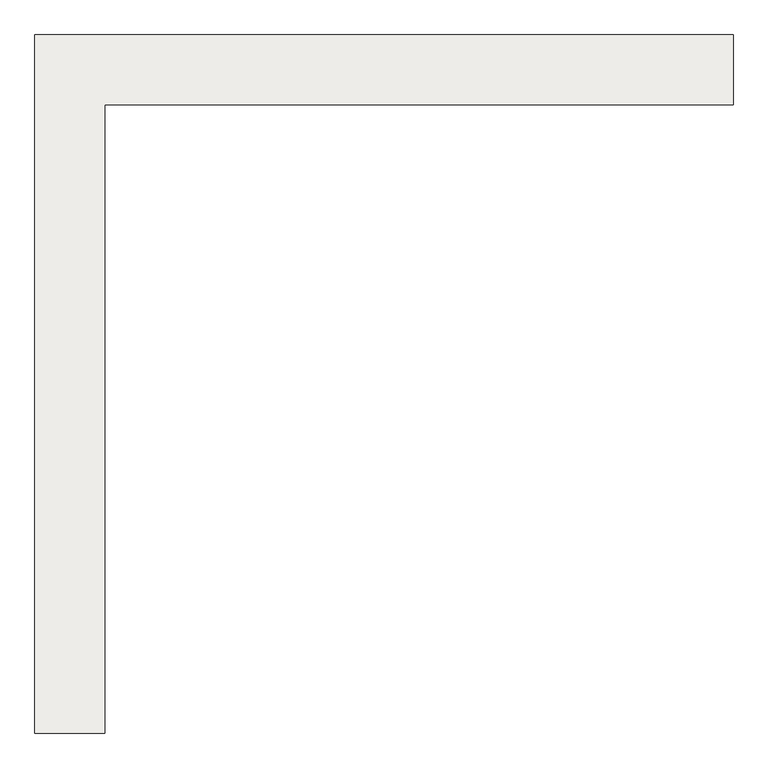
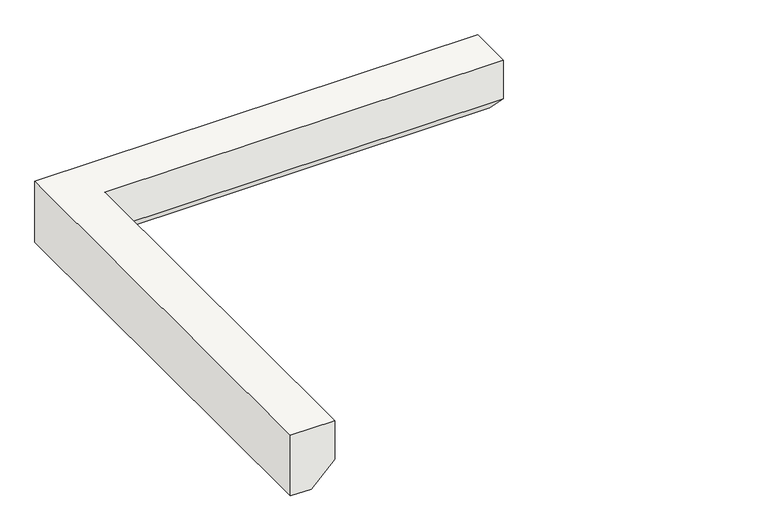
"""IFC4 building model written with IfcOpenShell, lengths in millimetres: slab geometry, hslab edge test : hslab edge test 1."""

from ifc_helpers import new_model, si_unit, origin, place, context, project, spatial, faceted_brep, source, transform, mapped, element, save


def slab_4663229b(model_context):
    return source(origin(), model_context, "Body", "Brep", [
        faceted_brep([(-959.1559606, 19799.5208589, -2020.0), (-959.1559606, 19799.5208589, -1800.0), (-1200.0, 19799.5208589, -1800.0), (-1200.0, 19799.5208589, -2147.2792206), (-1086.4351812, 19799.5208589, -2147.2792206), (-959.1559606, 21958.6768195, -2020.0), (-959.1559606, 21958.6768195, -1800.0), (1200.0, 21958.6768195, -1800.0), (1200.0, 22199.5208589, -1800.0), (-1200.0, 22199.5208589, -1800.0), (-1200.0, 22199.5208589, -2147.2792206), (1200.0, 22199.5208589, -2147.2792206), (1200.0, 22085.9560401, -2147.2792206), (-1086.4351812, 22085.9560401, -2147.2792206), (1200.0, 21958.6768195, -2020.0)], [[[0, 1, 2, 3, 4]], [[1, 0, 5, 6]], [[2, 1, 6, 7, 8, 9]], [[3, 2, 9, 10]], [[4, 3, 10, 11, 12, 13]], [[0, 4, 13, 5]], [[14, 12, 11, 8, 7]], [[6, 5, 14, 7]], [[10, 9, 8, 11]], [[5, 13, 12, 14]]]),
    ])


if __name__ == "__main__":
    model = new_model("IFC4")
    model_context = context("Model", 3, world=origin())
    ifc_project = project(units=[si_unit("LENGTHUNIT", "METRE", prefix="MILLI")], contexts=[model_context])
    site = spatial("IfcSite", under=ifc_project)
    building = spatial("IfcBuilding", under=site)
    placement = place(None, origin())
    slab_shape = slab_4663229b(model_context)
    element("IfcSlab", 1, ObjectType="hslab edge test : hslab edge test 1", at=placement, inside=building, context=model_context, shape_type="MappedRepresentation", body=[
        mapped(slab_shape, transform((0.0, 0.0, 0.0), x_axis=(1.0, 0.0, 0.0), y_axis=(0.0, 1.0, 0.0), z_axis=(0.0, 0.0, 1.0))),
    ])
    save(model, "model.ifc")
